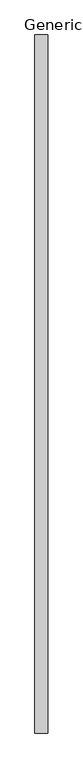
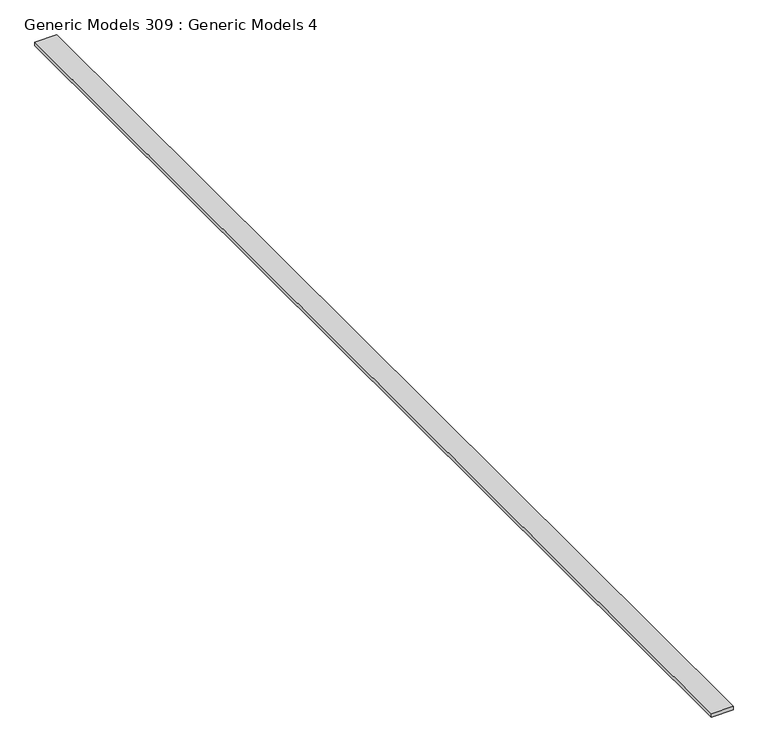
"""IFC4 building model written with IfcOpenShell, lengths in millimetres: proxy geometry, Generic Models 309 : Generic Models 4."""

from ifc_helpers import new_model, si_unit, frame, origin, place, context, project, spatial, polyline, outline, extrude, source, transform, mapped, element, save


def generic_models_309_generic_models_4_d66718fc(model_context):
    return source(origin(), model_context, "Body", "SweptSolid", [
        extrude(outline(polyline([(7338.4467872, -6864.9230338), (7223.4709223, -6864.9230338), (7223.4709223, -667.3230338), (7338.4467872, -667.3230338), (7338.4467872, -6864.9230338)])), frame((0.0, 0.0, 126524.8520404), z_axis=(0.0, 0.0, 1.0), x_axis=(1.0, 0.0, 0.0)), (0.0, 0.0, 1.0), 19.05),
    ])


if __name__ == "__main__":
    model = new_model("IFC4")
    model_context = context("Model", 3, world=origin())
    ifc_project = project(units=[si_unit("LENGTHUNIT", "METRE", prefix="MILLI")], contexts=[model_context])
    site = spatial("IfcSite", under=ifc_project)
    building = spatial("IfcBuilding", under=site)
    placement = place(None, origin())
    generic_models_309_generic_models_4_shape = generic_models_309_generic_models_4_d66718fc(model_context)
    element("IfcBuildingElementProxy", 1, Name="Generic Models 309 : Generic Models 4", ObjectType="Generic Models 309 : Generic Models 4", at=placement, inside=building, context=model_context, shape_type="MappedRepresentation", body=[
        mapped(generic_models_309_generic_models_4_shape, transform((0.0, 0.0, 0.0), x_axis=(1.0, 0.0, 0.0), y_axis=(0.0, 1.0, 0.0), z_axis=(0.0, 0.0, 1.0))),
    ])
    save(model, "model.ifc")

# Revit data of these elements
# Element 1 (IfcBuildingElementProxy, "Generic Models 309 : Generic Models 4")
#   Materials on its faces: "_CDX PLYWOOD - SEE STRUCT DWGs"
# Materials
#   "_CDX PLYWOOD - SEE STRUCT DWGs": class "Generic", colour RGB 98 75 74, transparency 0, Cost = 0
